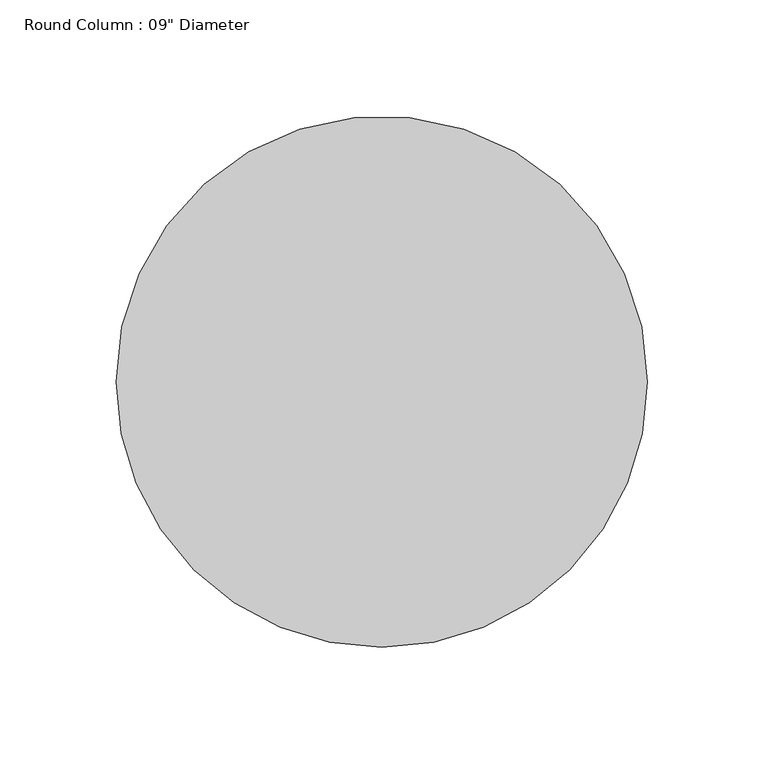
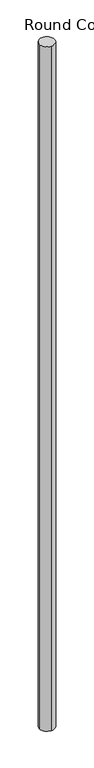
"""IFC4 building model written with IfcOpenShell, lengths in millimetres: column geometry."""

from ifc_helpers import new_model, si_unit, point, frame, origin, origin_2d, place, context, project, spatial, circle_curve, trimmed, segment, composite_curve, outline, extrude, source, transform, mapped, element, save


def column_45090e78(model_context):
    return source(origin(), model_context, "Body", "SweptSolid", [
        extrude(outline(composite_curve([segment(trimmed(circle_curve(origin_2d(), 114.3), [point((114.3, 0.0))], [point((0.0, -114.3))], False, "CARTESIAN"), True, "CONTINUOUS"), segment(trimmed(circle_curve(origin_2d(), 114.3), [point((0.0, -114.3))], [point((-114.3, 0.0))], False, "CARTESIAN"), True, "CONTINUOUS"), segment(trimmed(circle_curve(origin_2d(), 114.3), [point((-114.3, 0.0))], [point((114.3, 0.0))], False, "CARTESIAN"), True, "CONTINUOUS")], self_intersect=False)), frame((0.0, 0.0, 30327.6), z_axis=(0.0, 0.0, 1.0), x_axis=(1.0, 0.0, 0.0)), (0.0, 0.0, 1.0), 10922.0),
    ])


if __name__ == "__main__":
    model = new_model("IFC4")
    model_context = context("Model", 3, world=origin())
    ifc_project = project(units=[si_unit("LENGTHUNIT", "METRE", prefix="MILLI")], contexts=[model_context])
    site = spatial("IfcSite", under=ifc_project)
    building = spatial("IfcBuilding", under=site)
    placement = place(None, origin())
    column_shape = column_45090e78(model_context)
    element("IfcColumn", 1, ObjectType="Round Column : 09\" Diameter", at=placement, inside=building, context=model_context, shape_type="MappedRepresentation", body=[
        mapped(column_shape, transform((0.0, 0.0, 0.0), x_axis=(1.0, 0.0, 0.0), y_axis=(0.0, 1.0, 0.0), z_axis=(0.0, 0.0, 1.0))),
    ])
    save(model, "model.ifc")

# Revit data of these elements
# Type "Round Column : 09\" Diameter"
#   Assembly Code = "B1010200"
#   Diameter = 0' - 9"
#   Offset Base = 0' - 0"
#   Offset Top = 0' - 0"
#   Material = Metal - Aluminum
# Element 1 (IfcColumn, "Round Column : 09\" Diameter")
#   Materials on its faces: "Metal - Aluminum"
# Materials
#   "Metal - Aluminum": class "Metal", colour RGB 109 108 108, transparency 0
